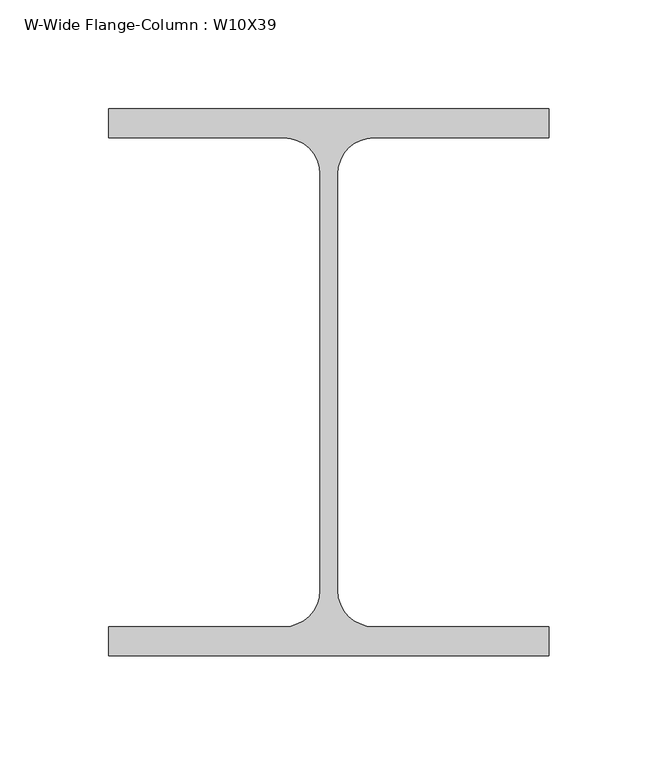
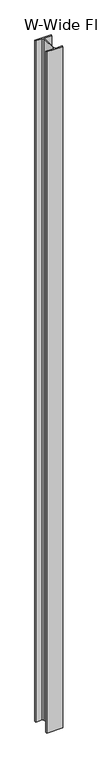
"""IFC4 building model written with IfcOpenShell, lengths in millimetres: column geometry, W-Wide Flange-Column : W10X39."""

from ifc_helpers import new_model, si_unit, point, frame, frame_2d, origin, place, context, project, spatial, polyline, circle_curve, trimmed, segment, composite_curve, outline, extrude, source, transform, mapped, element, save


def w_wide_flange_column_w10x39_5f667684(model_context):
    return source(origin(), model_context, "Body", "SweptSolid", [
        extrude(outline(composite_curve([segment(polyline([(101.473, 125.984), (101.473, 112.522), (20.701, 112.522)]), True, "CONTINUOUS"), segment(trimmed(circle_curve(frame_2d((20.701, 95.8215)), 16.7005), [point((20.701, 112.522))], [point((4.0005, 95.8215))], True, "CARTESIAN"), True, "CONTINUOUS"), segment(polyline([(4.0005, 95.8215), (4.0005, -95.8215)]), True, "CONTINUOUS"), segment(trimmed(circle_curve(frame_2d((20.701, -95.8215)), 16.7005), [point((4.0005, -95.8215))], [point((20.701, -112.522))], True, "CARTESIAN"), True, "CONTINUOUS"), segment(polyline([(20.701, -112.522), (101.473, -112.522), (101.473, -125.984), (-101.473, -125.984), (-101.473, -112.522), (-20.701, -112.522)]), True, "CONTINUOUS"), segment(trimmed(circle_curve(frame_2d((-20.701, -95.8215)), 16.7005), [point((-20.701, -112.522))], [point((-4.0005, -95.8215))], True, "CARTESIAN"), True, "CONTINUOUS"), segment(polyline([(-4.0005, -95.8215), (-4.0005, 95.8215)]), True, "CONTINUOUS"), segment(trimmed(circle_curve(frame_2d((-20.701, 95.8215)), 16.7005), [point((-4.0005, 95.8215))], [point((-20.701, 112.522))], True, "CARTESIAN"), True, "CONTINUOUS"), segment(polyline([(-20.701, 112.522), (-101.473, 112.522), (-101.473, 125.984), (101.473, 125.984)]), True, "CONTINUOUS")], self_intersect=False)), frame((0.0, 0.0, 8655.05), z_axis=(0.0, 0.0, 1.0), x_axis=(1.0, 0.0, 0.0)), (0.0, 0.0, 1.0), 8972.55),
    ])


if __name__ == "__main__":
    model = new_model("IFC4")
    model_context = context("Model", 3, world=origin())
    ifc_project = project(units=[si_unit("LENGTHUNIT", "METRE", prefix="MILLI")], contexts=[model_context])
    site = spatial("IfcSite", under=ifc_project)
    building = spatial("IfcBuilding", under=site)
    placement = place(None, origin())
    w_wide_flange_column_w10x39_shape = w_wide_flange_column_w10x39_5f667684(model_context)
    element("IfcColumn", 1, ObjectType="W-Wide Flange-Column : W10X39", at=placement, inside=building, context=model_context, shape_type="MappedRepresentation", body=[
        mapped(w_wide_flange_column_w10x39_shape, transform((0.0, 0.0, 0.0), x_axis=(1.0, 0.0, 0.0), y_axis=(0.0, 1.0, 0.0), z_axis=(0.0, 0.0, 1.0))),
    ])
    save(model, "model.ifc")

# Revit data of these elements
# Type "W-Wide Flange-Column : W10X39"
#   Assembly Code = "B10"
#   W = 39
#   bf = 0' - 7.99"
#   d = 0' - 9.92"
#   k = 0' - 1 3/16"
#   kr = 0' - 0.6575"
#   tf = 0' - 0.53"
#   tw = 0' - 0.315"
#   A = 0.0798611 SF
#   Structural Material [instance default] = Steel ASTM A992
# Element 1 (IfcColumn, "W-Wide Flange-Column : W10X39")
#   Materials on its faces: "Steel ASTM A992"
# Materials
#   "Steel ASTM A992": class "Metal", colour RGB 199 199 199, transparency 0, Description = "Structural steel 50ksi", Cost = 0
